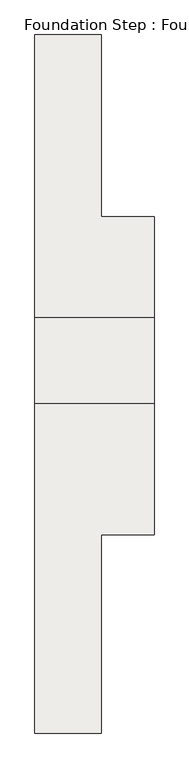
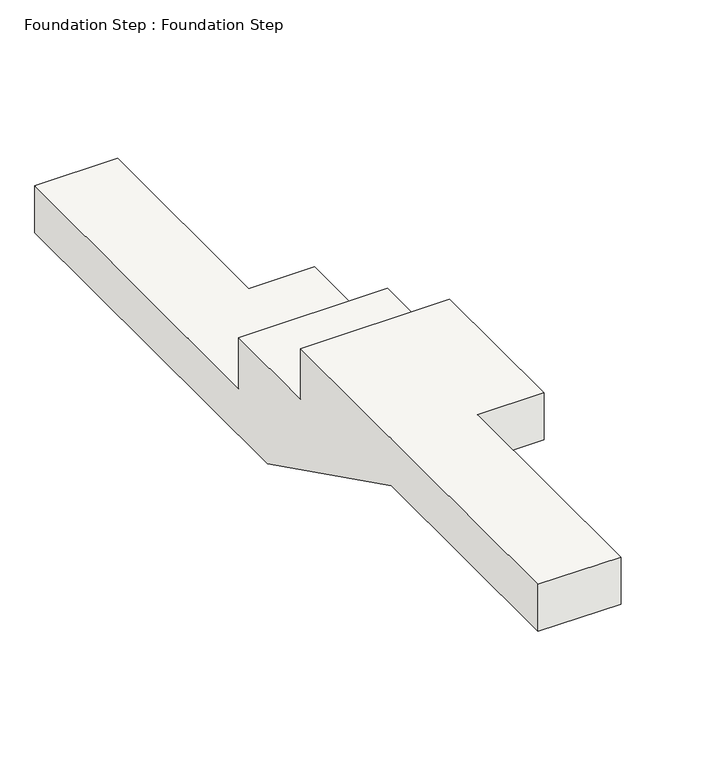
"""IFC4 building model written with IfcOpenShell, lengths in millimetres: slab geometry, Foundation Step : Foundation Step."""

from ifc_helpers import new_model, si_unit, origin, place, context, project, spatial, faceted_brep, source, transform, mapped, element, save


def foundation_step_foundation_step_6eb52276(model_context):
    return source(origin(), model_context, "Body", "Brep", [
        faceted_brep([(-65781.2850821, 11238.2505048, -1422.4), (-65781.2850821, 11238.2505048, -1752.6), (-65781.2850821, 13409.3518471, -1752.6), (-65781.2850821, 13409.3518471, -2057.4), (-65781.2850821, 10933.4505048, -2057.4), (-65781.2850821, 9612.6505048, -1397.0), (-65781.2850821, 8050.5505048, -1397.0), (-65781.2850821, 8050.5505048, -1092.2), (-65781.2850821, 10577.8505048, -1092.2), (-65781.2850821, 10577.8505048, -1422.4), (-64866.8850821, 11238.2505048, -1752.6), (-64866.8850821, 11238.2505048, -1422.4), (-64866.8850821, 10577.8505048, -1422.4), (-64866.8850821, 10577.8505048, -1092.2), (-64866.8850821, 9574.5505048, -1092.2), (-64866.8850821, 9574.5505048, -1397.0), (-64866.8850821, 9612.6505048, -1397.0), (-64866.8850821, 10933.4505048, -2057.4), (-64866.8850821, 12012.9505048, -2057.4), (-64866.8850821, 12012.9505048, -1752.6), (-65273.2850821, 12012.9505048, -1752.6), (-65273.2850821, 13409.3518471, -1752.6), (-65273.2850821, 13409.3518471, -2057.4), (-65273.2850821, 12012.9505048, -2057.4), (-65273.2850821, 9574.5505048, -1397.0), (-65273.2850821, 8050.5505048, -1397.0), (-65273.2850821, 8050.5505048, -1092.2), (-65273.2850821, 9574.5505048, -1092.2)], [[[0, 1, 2, 3, 4, 5, 6, 7, 8, 9]], [[10, 11, 12, 13, 14, 15, 16, 17, 18, 19]], [[1, 0, 11, 10]], [[2, 1, 10, 19, 20, 21]], [[3, 2, 21, 22]], [[4, 3, 22, 23, 18, 17]], [[6, 5, 16, 15, 24, 25]], [[7, 6, 25, 26]], [[8, 7, 26, 27, 14, 13]], [[9, 8, 13, 12]], [[0, 9, 12, 11]], [[5, 4, 17, 16]], [[27, 24, 15, 14]], [[24, 27, 26, 25]], [[20, 23, 22, 21]], [[23, 20, 19, 18]]]),
    ])


if __name__ == "__main__":
    model = new_model("IFC4")
    model_context = context("Model", 3, world=origin())
    ifc_project = project(units=[si_unit("LENGTHUNIT", "METRE", prefix="MILLI")], contexts=[model_context])
    site = spatial("IfcSite", under=ifc_project)
    building = spatial("IfcBuilding", under=site)
    placement = place(None, origin())
    foundation_step_foundation_step_shape = foundation_step_foundation_step_6eb52276(model_context)
    element("IfcSlab", 1, ObjectType="Foundation Step : Foundation Step", at=placement, inside=building, context=model_context, shape_type="MappedRepresentation", body=[
        mapped(foundation_step_foundation_step_shape, transform((0.0, 0.0, 0.0), x_axis=(1.0, 0.0, 0.0), y_axis=(0.0, 1.0, 0.0), z_axis=(0.0, 0.0, 1.0))),
    ])
    save(model, "model.ifc")

# Revit data of these elements
# Type "Foundation Step : Foundation Step"
#   Structural Material = Concrete, Cast-in-Place gray
# Materials
#   "Concrete, Cast-in-Place gray": class "Concrete", colour RGB 192 192 192, transparency 0, Description = "Cast-in-place concrete", Cost = 0
